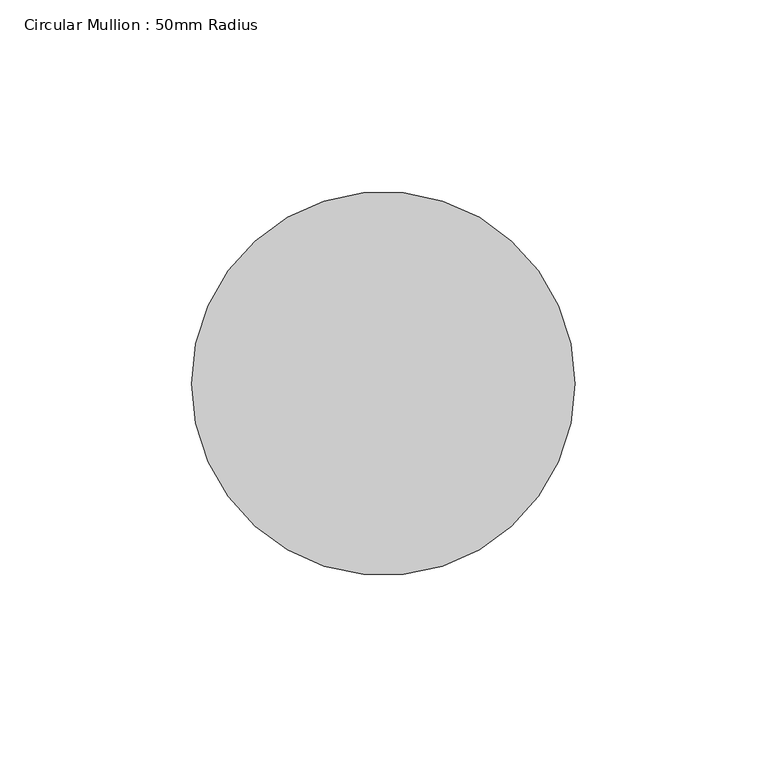
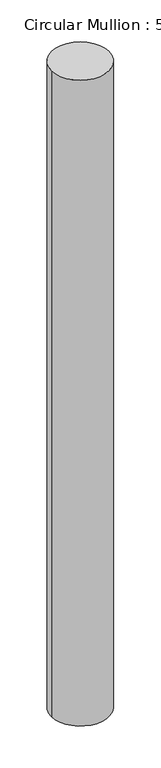
"""IFC4 building model written with IfcOpenShell, lengths in millimetres: member geometry, Circular Mullion : 50mm Radius."""

from ifc_helpers import new_model, si_unit, point, frame, origin, origin_2d, place, context, project, spatial, circle_curve, trimmed, segment, composite_curve, outline, extrude, source, transform, mapped, element, save


def circular_mullion_50mm_radius_284c2d69(model_context):
    return source(origin(), model_context, "Body", "SweptSolid", [
        extrude(outline(composite_curve([segment(trimmed(circle_curve(origin_2d(), 50.0), [point((50.0, 0.0))], [point((-50.0, 0.0))], False, "CARTESIAN"), True, "CONTINUOUS"), segment(trimmed(circle_curve(origin_2d(), 50.0), [point((-50.0, 0.0))], [point((50.0, 0.0))], False, "CARTESIAN"), True, "CONTINUOUS")], self_intersect=False)), frame((0.0, 0.0, -1181.1645788), z_axis=(0.0, 0.0, 1.0), x_axis=(1.0, 0.0, 0.0)), (0.0, 0.0, 1.0), 1181.1645788),
    ])


if __name__ == "__main__":
    model = new_model("IFC4")
    model_context = context("Model", 3, world=origin())
    ifc_project = project(units=[si_unit("LENGTHUNIT", "METRE", prefix="MILLI")], contexts=[model_context])
    site = spatial("IfcSite", under=ifc_project)
    building = spatial("IfcBuilding", under=site)
    placement = place(None, origin())
    circular_mullion_50mm_radius_shape = circular_mullion_50mm_radius_284c2d69(model_context)
    element("IfcMember", 1, ObjectType="Circular Mullion : 50mm Radius", at=placement, inside=building, context=model_context, shape_type="MappedRepresentation", body=[
        mapped(circular_mullion_50mm_radius_shape, transform((0.0, 0.0, 0.0), x_axis=(1.0, 0.0, 0.0), y_axis=(0.0, 1.0, 0.0), z_axis=(0.0, 0.0, 1.0))),
    ])
    save(model, "model.ifc")

# Revit data of these elements
# Type "Circular Mullion : 50mm Radius"
#   built-in parameter 1007350 = 0.164042 (stored number, unit not read)
# Element 1 (IfcMember, "Circular Mullion : 50mm Radius")
#   Materials on its faces: "Aluminium"
# Materials
#   "Aluminium": class "Metal", colour RGB 247 247 247, transparency 0, Description = "Aluminium 6061", Cost = 0
